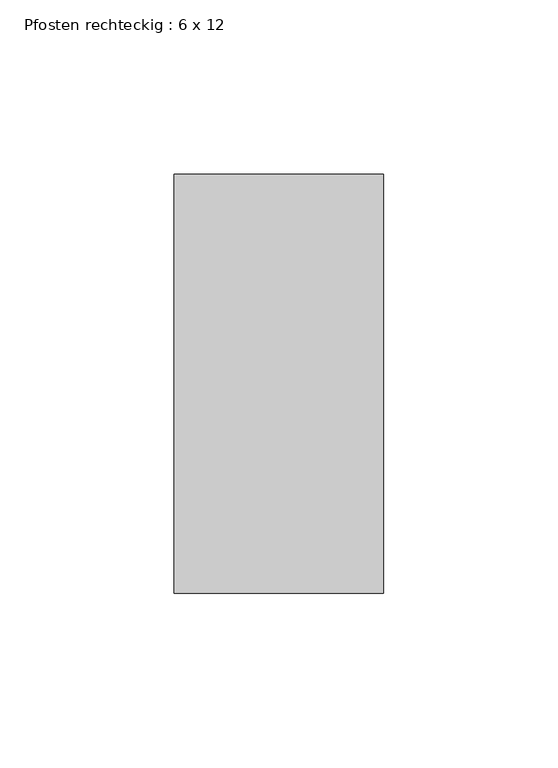
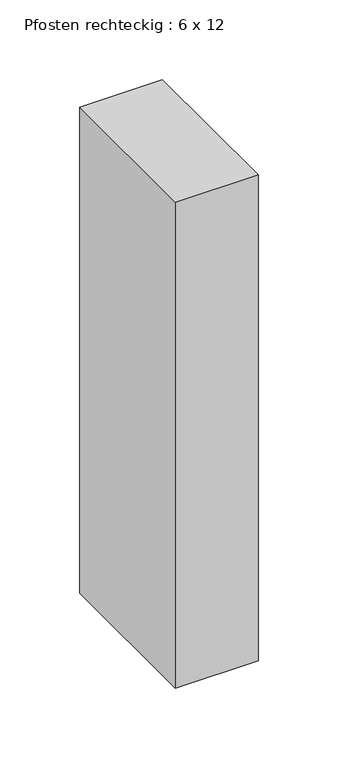
"""IFC4 building model written with IfcOpenShell, lengths in millimetres: member geometry, Pfosten rechteckig : 6 x 12."""

from ifc_helpers import new_model, si_unit, frame, origin, place, context, project, spatial, polyline, outline, extrude, source, transform, mapped, element, save


def pfosten_rechteckig_6_x_12_4751e821(model_context):
    return source(origin(), model_context, "Body", "SweptSolid", [
        extrude(outline(polyline([(0.0, 60.0), (0.0, -60.0), (-60.0, -60.0), (-60.0, 60.0), (0.0, 60.0)])), frame((0.0, 0.0, -372.4999997), z_axis=(0.0, 0.0, 1.0), x_axis=(1.0, 0.0, 0.0)), (0.0, 0.0, 1.0), 372.4999997),
    ])


if __name__ == "__main__":
    model = new_model("IFC4")
    model_context = context("Model", 3, world=origin())
    ifc_project = project(units=[si_unit("LENGTHUNIT", "METRE", prefix="MILLI")], contexts=[model_context])
    site = spatial("IfcSite", under=ifc_project)
    building = spatial("IfcBuilding", under=site)
    placement = place(None, origin())
    pfosten_rechteckig_6_x_12_shape = pfosten_rechteckig_6_x_12_4751e821(model_context)
    element("IfcMember", 1, ObjectType="Pfosten rechteckig : 6 x 12", at=placement, inside=building, context=model_context, shape_type="MappedRepresentation", body=[
        mapped(pfosten_rechteckig_6_x_12_shape, transform((0.0, 0.0, 0.0), x_axis=(1.0, 0.0, 0.0), y_axis=(0.0, 1.0, 0.0), z_axis=(0.0, 0.0, 1.0))),
    ])
    save(model, "model.ifc")

# Revit data of these elements
# Type "Pfosten rechteckig : 6 x 12"
#   built-in parameter 1007304 = 0.393701 (stored number, unit not read)
#   built-in parameter 1007301 = 0.0984252 (stored number, unit not read)
#   built-in parameter 1007300 = 0.0984252 (stored number, unit not read)
# Element 1 (IfcMember, "Pfosten rechteckig : 6 x 12")
#   Materials on its faces: "Metall - verzinkt"
# Materials
#   "Metall - verzinkt": class "Allgemeines", colour RGB 200 200 200, transparency 0, Cost = 0
